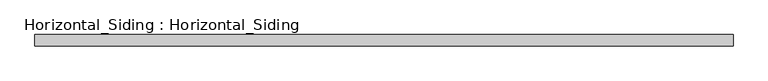
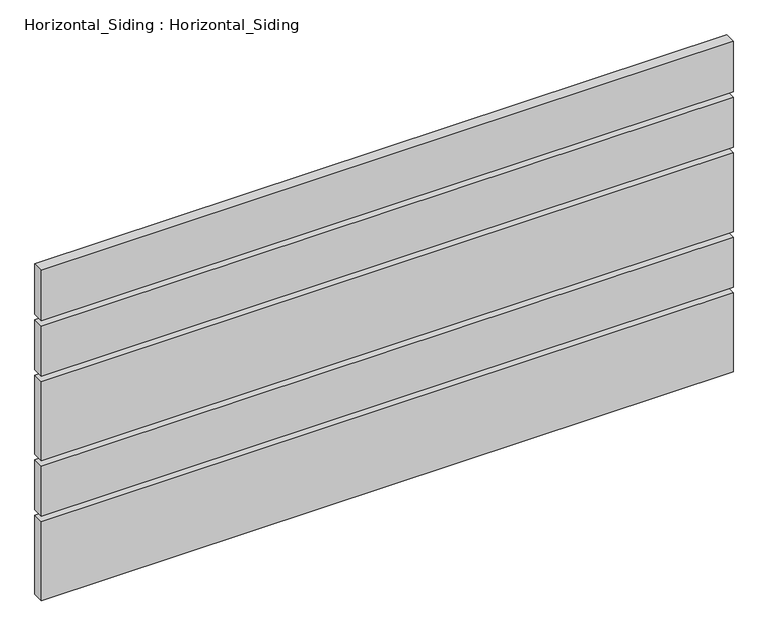
"""IFC4 building model written with IfcOpenShell, lengths in millimetres: plate geometry, Horizontal_Siding : Horizontal_Siding."""

import ifcopenshell
import ifcopenshell.guid

model = None  # the IFC model being written
_history = None  # IfcOwnerHistory: only IFC2X3 demands one
_inside = {}  # id of a spatial element -> (the spatial element, [elements in it])
_under = {}  # id of a project, library or spatial element -> (it, [spatial elements below it])
_declared = {}  # id of a project -> (the project, [libraries it declares])
_typed = {}  # id of a type object -> (the type object, [elements of that type])
_made_of = {}  # id of a material, layer set ... -> (it, [elements and type objects made of it])


def new_model(schema):
    """Start an empty IFC model of exactly this schema.

    Asked for "IFC4X3", IfcOpenShell would pick the latest addendum, in which some entities
    have other attributes; the version numbers below select the first issue.
    IFC2X3 requires an IfcOwnerHistory on every rooted entity: one is made here for all.
    """
    global model, _history
    if schema == "IFC4X3":
        model = ifcopenshell.file(schema_version=(4, 3, 0, 0))
    else:
        model = ifcopenshell.file(schema=schema)
    _inside.clear()
    _under.clear()
    _declared.clear()
    _typed.clear()
    _made_of.clear()
    _history = None
    if model.schema == "IFC2X3":
        org = make("IfcOrganization", Name="unknown")
        user = make(
            "IfcPersonAndOrganization",
            ThePerson=make("IfcPerson", FamilyName="unknown"),
            TheOrganization=org,
        )
        app = make(
            "IfcApplication",
            ApplicationDeveloper=org,
            Version="unknown",
            ApplicationFullName="unknown",
            ApplicationIdentifier="unknown",
        )
        _history = make(
            "IfcOwnerHistory",
            OwningUser=user,
            OwningApplication=app,
            ChangeAction="ADDED",
            CreationDate=0,
        )
    return model


def make(cls, **values):
    """One entity of the class cls with the attributes given. An attribute that is None is left unset."""
    return model.create_entity(
        cls, **{name: value for name, value in values.items() if value is not None}
    )


def rooted(cls, **values):
    """An entity with a GlobalId (a new one), such as an element, a storey or a relation."""
    return make(cls, GlobalId=ifcopenshell.guid.new(), OwnerHistory=_history, **values)


def si_unit(unit_type, name, prefix=None):
    """IfcSIUnit, for example si_unit("LENGTHUNIT", "METRE", prefix="MILLI")."""
    return make("IfcSIUnit", UnitType=unit_type, Prefix=prefix, Name=name)


def assignment(units):
    """IfcUnitAssignment: the units of a project."""
    return None if units is None else make("IfcUnitAssignment", Units=units)


def point(xyz):
    """IfcCartesianPoint."""
    return None if xyz is None else make("IfcCartesianPoint", Coordinates=xyz)


def direction(xyz):
    """IfcDirection."""
    return None if xyz is None else make("IfcDirection", DirectionRatios=xyz)


def frame(location, z_axis=None, x_axis=None):
    """IfcAxis2Placement3D, a coordinate frame: its origin and axes. An axis left out is left unset."""
    return make(
        "IfcAxis2Placement3D",
        Location=point(location),
        Axis=direction(z_axis),
        RefDirection=direction(x_axis),
    )


def origin():
    """The frame at (0, 0, 0) with its axes left unset."""
    return frame((0.0, 0.0, 0.0))


def place(relative_to, where):
    """IfcLocalPlacement: puts the frame where relative to a parent placement (None: the world)."""
    return make(
        "IfcLocalPlacement", PlacementRelTo=relative_to, RelativePlacement=where
    )


def context(
    kind, dimensions, precision=None, world=None, true_north=None, identifier=None
):
    """IfcGeometricRepresentationContext, for example the 3D "Model" context."""
    return make(
        "IfcGeometricRepresentationContext",
        ContextIdentifier=identifier,
        ContextType=kind,
        CoordinateSpaceDimension=dimensions,
        Precision=precision,
        WorldCoordinateSystem=world,
        TrueNorth=true_north,
    )


def project(units=None, contexts=None):
    """IfcProject with its units and contexts."""
    return rooted(
        "IfcProject",
        Name="project",
        RepresentationContexts=contexts,
        UnitsInContext=assignment(units),
    )


def spatial(cls, under=None, at=None, **own):
    """A site, building, storey or space (cls), placed at a placement, below another one or the project."""
    s = rooted(cls, ObjectPlacement=at, **own)
    if under is not None:
        _under.setdefault(under.id(), (under, []))[1].append(s)
    return s


def polyline(points):
    """IfcPolyline through the points."""
    return make("IfcPolyline", Points=[point(p) for p in points])


def outline(outer, holes=None, kind="AREA"):
    """IfcArbitraryClosedProfileDef: a profile drawn as a closed curve; with holes, ...WithVoids."""
    if holes is None:
        return make("IfcArbitraryClosedProfileDef", ProfileType=kind, OuterCurve=outer)
    return make(
        "IfcArbitraryProfileDefWithVoids",
        ProfileType=kind,
        OuterCurve=outer,
        InnerCurves=holes,
    )


def extrude(swept, where, along, depth):
    """IfcExtrudedAreaSolid: the profile swept, set in the frame where, extruded along a direction by depth."""
    return make(
        "IfcExtrudedAreaSolid",
        SweptArea=swept,
        Position=where,
        ExtrudedDirection=direction(along),
        Depth=depth,
    )


def shape(context_of_items, identifier, shape_type, items):
    """IfcShapeRepresentation: the items that make up one representation, for example the "Body"."""
    return make(
        "IfcShapeRepresentation",
        ContextOfItems=context_of_items,
        RepresentationIdentifier=identifier,
        RepresentationType=shape_type,
        Items=items,
    )


def source(mapping_origin, context_of_items, identifier, shape_type, items):
    """IfcRepresentationMap: a shape defined once, which mapped items show again and again."""
    return make(
        "IfcRepresentationMap",
        MappingOrigin=mapping_origin,
        MappedRepresentation=shape(context_of_items, identifier, shape_type, items),
    )


def transform(
    local_origin,
    x_axis=None,
    y_axis=None,
    z_axis=None,
    scale=None,
    scale2=None,
    scale3=None,
    uniform=True,
):
    """IfcCartesianTransformationOperator3D, or its non-uniform kind. x_axis, y_axis, z_axis: its Axis1, 2, 3."""
    if uniform:
        return make(
            "IfcCartesianTransformationOperator3D",
            Axis1=direction(x_axis),
            Axis2=direction(y_axis),
            LocalOrigin=point(local_origin),
            Scale=scale,
            Axis3=direction(z_axis),
        )
    return make(
        "IfcCartesianTransformationOperator3DnonUniform",
        Axis1=direction(x_axis),
        Axis2=direction(y_axis),
        LocalOrigin=point(local_origin),
        Scale=scale,
        Axis3=direction(z_axis),
        Scale2=scale2,
        Scale3=scale3,
    )


def mapped(mapping_source, mapping_target):
    """IfcMappedItem: shows the shape of a source again, moved by a transform."""
    return make(
        "IfcMappedItem", MappingSource=mapping_source, MappingTarget=mapping_target
    )


def made_of(thing, what):
    """Note that an element or type object is made of a material, layer set ...; save() writes the relation."""
    if what is not None:
        _made_of.setdefault(what.id(), (what, []))[1].append(thing)
    return thing


def element(
    cls,
    number,
    at=None,
    inside=None,
    cuts=None,
    type_object=None,
    material=None,
    context=None,
    identifier="Body",
    shape_type=None,
    held_by="IfcProductDefinitionShape",
    body=None,
    shapes=None,
    **own,
):
    """One element of the class cls, such as IfcWall. Its Tag is "e" and its number.

    at: its placement. inside: the storey or other place that contains it. cuts: it is an
    opening in that element (IfcRelVoidsElement). A single representation is given by context,
    identifier, shape_type and body (its items); several are given by shapes. held_by: the class
    of the entity that holds the representations. save() writes the other relations.
    """
    e = rooted(cls, Tag="e%d" % number, ObjectPlacement=at, **own)
    if body is not None:
        shapes = [shape(context, identifier, shape_type, body)]
    if shapes is not None:
        e.Representation = make(held_by, Representations=shapes)
    if inside is not None:
        _inside.setdefault(inside.id(), (inside, []))[1].append(e)
    if cuts is not None:
        rooted(
            "IfcRelVoidsElement", RelatingBuildingElement=cuts, RelatedOpeningElement=e
        )
    if type_object is not None:
        _typed.setdefault(type_object.id(), (type_object, []))[1].append(e)
    return made_of(e, material)


def aggregate(whole, parts):
    """IfcRelAggregates: a whole, such as a stair, and the parts it consists of."""
    return rooted("IfcRelAggregates", RelatingObject=whole, RelatedObjects=parts)


def save(model, path):
    """Write the relations noted so far, then the file.

    IfcRelAggregates (storeys below a building ...), IfcRelContainedInSpatialStructure (elements
    in a storey), IfcRelDefinesByType, IfcRelAssociatesMaterial and IfcRelDeclares: one each for
    every whole, place, type object, material and project.
    """
    for whole, parts in _under.values():
        aggregate(whole, parts)
    for where, things in _inside.values():
        rooted(
            "IfcRelContainedInSpatialStructure",
            RelatedElements=things,
            RelatingStructure=where,
        )
    for kind, things in _typed.values():
        rooted("IfcRelDefinesByType", RelatedObjects=things, RelatingType=kind)
    for what, things in _made_of.values():
        rooted("IfcRelAssociatesMaterial", RelatedObjects=things, RelatingMaterial=what)
    for by, libraries in _declared.values():
        rooted("IfcRelDeclares", RelatingContext=by, RelatedDefinitions=libraries)
    model.write(path)


def horizontal_siding_horizontal_siding_0b0f6f12(model_context):
    return source(origin(), model_context, "Body", "SweptSolid", [
        extrude(outline(polyline([(578.64375, -19.05), (-578.64375, -19.05), (-578.64375, 0.0), (578.64375, 0.0), (578.64375, -19.05)])), frame((0.0, 0.0, 9.525), z_axis=(0.0, 0.0, 1.0), x_axis=(1.0, 0.0, 0.0)), (0.0, 0.0, 1.0), 139.7),
        extrude(outline(polyline([(578.64375, -19.05), (-578.64375, -19.05), (-578.64375, 0.0), (578.64375, 0.0), (578.64375, -19.05)])), frame((0.0, 0.0, 158.75), z_axis=(0.0, 0.0, 1.0), x_axis=(1.0, 0.0, 0.0)), (0.0, 0.0, 1.0), 88.9),
        extrude(outline(polyline([(578.64375, -19.05), (-578.64375, -19.05), (-578.64375, 0.0), (578.64375, 0.0), (578.64375, -19.05)])), frame((0.0, 0.0, 257.175), z_axis=(0.0, 0.0, 1.0), x_axis=(1.0, 0.0, 0.0)), (0.0, 0.0, 1.0), 139.7),
        extrude(outline(polyline([(578.64375, -19.05), (-578.64375, -19.05), (-578.64375, 0.0), (578.64375, 0.0), (578.64375, -19.05)])), frame((0.0, 0.0, 406.4), z_axis=(0.0, 0.0, 1.0), x_axis=(1.0, 0.0, 0.0)), (0.0, 0.0, 1.0), 88.9),
        extrude(outline(polyline([(578.64375, -19.05), (-578.64375, -19.05), (-578.64375, 0.0), (578.64375, 0.0), (578.64375, -19.05)])), frame((0.0, 0.0, 504.825), z_axis=(0.0, 0.0, 1.0), x_axis=(1.0, 0.0, 0.0)), (0.0, 0.0, 1.0), 88.9),
    ])


if __name__ == "__main__":
    model = new_model("IFC4")
    model_context = context("Model", 3, world=origin())
    ifc_project = project(units=[si_unit("LENGTHUNIT", "METRE", prefix="MILLI")], contexts=[model_context])
    site = spatial("IfcSite", under=ifc_project)
    building = spatial("IfcBuilding", under=site)
    placement = place(None, origin())
    horizontal_siding_horizontal_siding_shape = horizontal_siding_horizontal_siding_0b0f6f12(model_context)
    element("IfcPlate", 1, ObjectType="Horizontal_Siding : Horizontal_Siding", at=placement, inside=building, context=model_context, shape_type="MappedRepresentation", body=[
        mapped(horizontal_siding_horizontal_siding_shape, transform((0.0, 0.0, 0.0), x_axis=(1.0, 0.0, 0.0), y_axis=(0.0, 1.0, 0.0), z_axis=(0.0, 0.0, 1.0))),
    ])
    save(model, "model.ifc")

# Revit data of these elements
# Type "Horizontal_Siding : Horizontal_Siding"
#   Analytic Construction = "<None>"
#   extend = 0' - 2 3/4"
#   Width_2 = 0' - 3 1/2"
#   Width_1 = 0' - 5 1/2"
#   Gap = 0' - 0 3/8"
#   Plank Material = SLOTTED WOOD FENCE (THERMALLY MODIFIED WOOD: ARBOR WOOD)\n(EXTERIOR STAIN : PENOFIN VERDE EXT. STAIN - COLOR: CEDAR)
# Element 1 (IfcPlate, "Horizontal_Siding : Horizontal_Siding")
#   Materials on its faces: "SLOTTED WOOD FENCE (THERMALLY MODIFIED WOOD: ARBOR WOOD)\n(EXTERIOR STAIN : PENOFIN VERDE EXT. STAIN - COLOR: CEDAR)"
# Materials
#   "SLOTTED WOOD FENCE (THERMALLY MODIFIED WOOD: ARBOR WOOD)\n(EXTERIOR STAIN : PENOFIN VERDE EXT. STAIN - COLOR: CEDAR)": class "Wood", colour RGB 164 134 123, transparency 0, Description = "Pinus Echinata", Cost = 0
